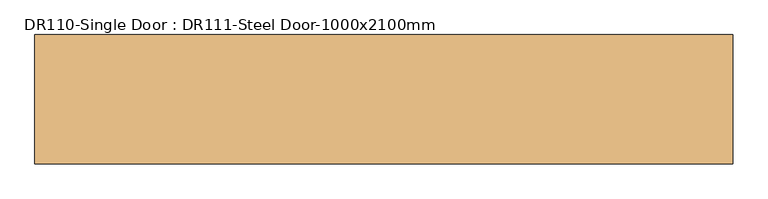
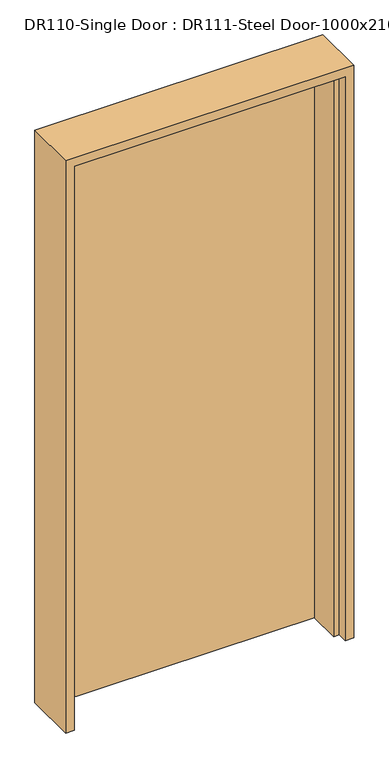
"""IFC4 building model written with IfcOpenShell, lengths in millimetres: door geometry, DR110-Single Door : DR111-Steel Door-1000x2100mm."""

import ifcopenshell
import ifcopenshell.guid

model = None  # the IFC model being written
_history = None  # IfcOwnerHistory: only IFC2X3 demands one
_inside = {}  # id of a spatial element -> (the spatial element, [elements in it])
_under = {}  # id of a project, library or spatial element -> (it, [spatial elements below it])
_declared = {}  # id of a project -> (the project, [libraries it declares])
_typed = {}  # id of a type object -> (the type object, [elements of that type])
_made_of = {}  # id of a material, layer set ... -> (it, [elements and type objects made of it])


def new_model(schema):
    """Start an empty IFC model of exactly this schema.

    Asked for "IFC4X3", IfcOpenShell would pick the latest addendum, in which some entities
    have other attributes; the version numbers below select the first issue.
    IFC2X3 requires an IfcOwnerHistory on every rooted entity: one is made here for all.
    """
    global model, _history
    if schema == "IFC4X3":
        model = ifcopenshell.file(schema_version=(4, 3, 0, 0))
    else:
        model = ifcopenshell.file(schema=schema)
    _inside.clear()
    _under.clear()
    _declared.clear()
    _typed.clear()
    _made_of.clear()
    _history = None
    if model.schema == "IFC2X3":
        org = make("IfcOrganization", Name="unknown")
        user = make(
            "IfcPersonAndOrganization",
            ThePerson=make("IfcPerson", FamilyName="unknown"),
            TheOrganization=org,
        )
        app = make(
            "IfcApplication",
            ApplicationDeveloper=org,
            Version="unknown",
            ApplicationFullName="unknown",
            ApplicationIdentifier="unknown",
        )
        _history = make(
            "IfcOwnerHistory",
            OwningUser=user,
            OwningApplication=app,
            ChangeAction="ADDED",
            CreationDate=0,
        )
    return model


def make(cls, **values):
    """One entity of the class cls with the attributes given. An attribute that is None is left unset."""
    return model.create_entity(
        cls, **{name: value for name, value in values.items() if value is not None}
    )


def rooted(cls, **values):
    """An entity with a GlobalId (a new one), such as an element, a storey or a relation."""
    return make(cls, GlobalId=ifcopenshell.guid.new(), OwnerHistory=_history, **values)


def si_unit(unit_type, name, prefix=None):
    """IfcSIUnit, for example si_unit("LENGTHUNIT", "METRE", prefix="MILLI")."""
    return make("IfcSIUnit", UnitType=unit_type, Prefix=prefix, Name=name)


def assignment(units):
    """IfcUnitAssignment: the units of a project."""
    return None if units is None else make("IfcUnitAssignment", Units=units)


def point(xyz):
    """IfcCartesianPoint."""
    return None if xyz is None else make("IfcCartesianPoint", Coordinates=xyz)


def direction(xyz):
    """IfcDirection."""
    return None if xyz is None else make("IfcDirection", DirectionRatios=xyz)


def frame(location, z_axis=None, x_axis=None):
    """IfcAxis2Placement3D, a coordinate frame: its origin and axes. An axis left out is left unset."""
    return make(
        "IfcAxis2Placement3D",
        Location=point(location),
        Axis=direction(z_axis),
        RefDirection=direction(x_axis),
    )


def origin():
    """The frame at (0, 0, 0) with its axes left unset."""
    return frame((0.0, 0.0, 0.0))


def origin_with_axes():
    """The frame at (0, 0, 0) with the z axis (0, 0, 1) and the x axis (1, 0, 0) written out."""
    return frame((0.0, 0.0, 0.0), z_axis=(0.0, 0.0, 1.0), x_axis=(1.0, 0.0, 0.0))


def place(relative_to, where):
    """IfcLocalPlacement: puts the frame where relative to a parent placement (None: the world)."""
    return make(
        "IfcLocalPlacement", PlacementRelTo=relative_to, RelativePlacement=where
    )


def context(
    kind, dimensions, precision=None, world=None, true_north=None, identifier=None
):
    """IfcGeometricRepresentationContext, for example the 3D "Model" context."""
    return make(
        "IfcGeometricRepresentationContext",
        ContextIdentifier=identifier,
        ContextType=kind,
        CoordinateSpaceDimension=dimensions,
        Precision=precision,
        WorldCoordinateSystem=world,
        TrueNorth=true_north,
    )


def project(units=None, contexts=None):
    """IfcProject with its units and contexts."""
    return rooted(
        "IfcProject",
        Name="project",
        RepresentationContexts=contexts,
        UnitsInContext=assignment(units),
    )


def spatial(cls, under=None, at=None, **own):
    """A site, building, storey or space (cls), placed at a placement, below another one or the project."""
    s = rooted(cls, ObjectPlacement=at, **own)
    if under is not None:
        _under.setdefault(under.id(), (under, []))[1].append(s)
    return s


def polyline(points):
    """IfcPolyline through the points."""
    return make("IfcPolyline", Points=[point(p) for p in points])


def outline(outer, holes=None, kind="AREA"):
    """IfcArbitraryClosedProfileDef: a profile drawn as a closed curve; with holes, ...WithVoids."""
    if holes is None:
        return make("IfcArbitraryClosedProfileDef", ProfileType=kind, OuterCurve=outer)
    return make(
        "IfcArbitraryProfileDefWithVoids",
        ProfileType=kind,
        OuterCurve=outer,
        InnerCurves=holes,
    )


def extrude(swept, where, along, depth):
    """IfcExtrudedAreaSolid: the profile swept, set in the frame where, extruded along a direction by depth."""
    return make(
        "IfcExtrudedAreaSolid",
        SweptArea=swept,
        Position=where,
        ExtrudedDirection=direction(along),
        Depth=depth,
    )


def faces_of(points, faces, orient=None, outer=None):
    """IfcFace entities. A face is a list of loops; a loop is a list of indices into points, from 0.

    orient and outer hold one flag for each loop. By default every Orientation is true, the
    first loop of a face is its IfcFaceOuterBound and the others are IfcFaceBound.
    """
    made = []
    for i, loops in enumerate(faces):
        bounds = []
        for j, loop in enumerate(loops):
            is_outer = j == 0 if outer is None else outer[i][j]
            bounds.append(
                make(
                    "IfcFaceOuterBound" if is_outer else "IfcFaceBound",
                    Bound=make("IfcPolyLoop", Polygon=[points[k] for k in loop]),
                    Orientation=True if orient is None else orient[i][j],
                )
            )
        made.append(make("IfcFace", Bounds=bounds))
    return made


def faceted_brep(points, faces, orient=None, outer=None, voids=None):
    """IfcFacetedBrep: a solid bounded by flat faces; with voids (closed shells), ...WithVoids."""
    shared = [point(p) for p in points]
    hull = make("IfcClosedShell", CfsFaces=faces_of(shared, faces, orient, outer))
    if voids is None:
        return make("IfcFacetedBrep", Outer=hull)
    return make(
        "IfcFacetedBrepWithVoids",
        Outer=hull,
        Voids=[
            make(cls, CfsFaces=faces_of(shared, fs, o, b)) for cls, fs, o, b in voids
        ],
    )


def shape(context_of_items, identifier, shape_type, items):
    """IfcShapeRepresentation: the items that make up one representation, for example the "Body"."""
    return make(
        "IfcShapeRepresentation",
        ContextOfItems=context_of_items,
        RepresentationIdentifier=identifier,
        RepresentationType=shape_type,
        Items=items,
    )


def source(mapping_origin, context_of_items, identifier, shape_type, items):
    """IfcRepresentationMap: a shape defined once, which mapped items show again and again."""
    return make(
        "IfcRepresentationMap",
        MappingOrigin=mapping_origin,
        MappedRepresentation=shape(context_of_items, identifier, shape_type, items),
    )


def transform(
    local_origin,
    x_axis=None,
    y_axis=None,
    z_axis=None,
    scale=None,
    scale2=None,
    scale3=None,
    uniform=True,
):
    """IfcCartesianTransformationOperator3D, or its non-uniform kind. x_axis, y_axis, z_axis: its Axis1, 2, 3."""
    if uniform:
        return make(
            "IfcCartesianTransformationOperator3D",
            Axis1=direction(x_axis),
            Axis2=direction(y_axis),
            LocalOrigin=point(local_origin),
            Scale=scale,
            Axis3=direction(z_axis),
        )
    return make(
        "IfcCartesianTransformationOperator3DnonUniform",
        Axis1=direction(x_axis),
        Axis2=direction(y_axis),
        LocalOrigin=point(local_origin),
        Scale=scale,
        Axis3=direction(z_axis),
        Scale2=scale2,
        Scale3=scale3,
    )


def mapped(mapping_source, mapping_target):
    """IfcMappedItem: shows the shape of a source again, moved by a transform."""
    return make(
        "IfcMappedItem", MappingSource=mapping_source, MappingTarget=mapping_target
    )


def made_of(thing, what):
    """Note that an element or type object is made of a material, layer set ...; save() writes the relation."""
    if what is not None:
        _made_of.setdefault(what.id(), (what, []))[1].append(thing)
    return thing


def element(
    cls,
    number,
    at=None,
    inside=None,
    cuts=None,
    type_object=None,
    material=None,
    context=None,
    identifier="Body",
    shape_type=None,
    held_by="IfcProductDefinitionShape",
    body=None,
    shapes=None,
    **own,
):
    """One element of the class cls, such as IfcWall. Its Tag is "e" and its number.

    at: its placement. inside: the storey or other place that contains it. cuts: it is an
    opening in that element (IfcRelVoidsElement). A single representation is given by context,
    identifier, shape_type and body (its items); several are given by shapes. held_by: the class
    of the entity that holds the representations. save() writes the other relations.
    """
    e = rooted(cls, Tag="e%d" % number, ObjectPlacement=at, **own)
    if body is not None:
        shapes = [shape(context, identifier, shape_type, body)]
    if shapes is not None:
        e.Representation = make(held_by, Representations=shapes)
    if inside is not None:
        _inside.setdefault(inside.id(), (inside, []))[1].append(e)
    if cuts is not None:
        rooted(
            "IfcRelVoidsElement", RelatingBuildingElement=cuts, RelatedOpeningElement=e
        )
    if type_object is not None:
        _typed.setdefault(type_object.id(), (type_object, []))[1].append(e)
    return made_of(e, material)


def aggregate(whole, parts):
    """IfcRelAggregates: a whole, such as a stair, and the parts it consists of."""
    return rooted("IfcRelAggregates", RelatingObject=whole, RelatedObjects=parts)


def save(model, path):
    """Write the relations noted so far, then the file.

    IfcRelAggregates (storeys below a building ...), IfcRelContainedInSpatialStructure (elements
    in a storey), IfcRelDefinesByType, IfcRelAssociatesMaterial and IfcRelDeclares: one each for
    every whole, place, type object, material and project.
    """
    for whole, parts in _under.values():
        aggregate(whole, parts)
    for where, things in _inside.values():
        rooted(
            "IfcRelContainedInSpatialStructure",
            RelatedElements=things,
            RelatingStructure=where,
        )
    for kind, things in _typed.values():
        rooted("IfcRelDefinesByType", RelatedObjects=things, RelatingType=kind)
    for what, things in _made_of.values():
        rooted("IfcRelAssociatesMaterial", RelatedObjects=things, RelatingMaterial=what)
    for by, libraries in _declared.values():
        rooted("IfcRelDeclares", RelatingContext=by, RelatedDefinitions=libraries)
    model.write(path)


def dr110_single_door_dr111_steel_door_1000x2100mm_0699664c(model_context):
    return source(origin(), model_context, "Body", "SolidModel", [
        extrude(outline(polyline([(470.0, 92.5), (470.0, 57.5), (-470.0, 57.5), (-470.0, 92.5), (470.0, 92.5)])), origin_with_axes(), (0.0, 0.0, 1.0), 2070.0),
        faceted_brep([(470.0, 92.5, 0.0), (500.0, 92.5, 0.0), (500.0, -92.5, 0.0), (470.0, -92.5, 0.0), (470.0, -57.5, 0.0), (450.0, -57.5, 0.0), (450.0, 57.5, 0.0), (470.0, 57.5, 0.0), (470.0, 92.5, 2070.0), (-470.0, 92.5, 2070.0), (-470.0, 92.5, 0.0), (-500.0, 92.5, 0.0), (-500.0, 92.5, 2100.0), (500.0, 92.5, 2100.0), (500.0, -92.5, 2100.0), (-500.0, -92.5, 2100.0), (-500.0, -92.5, 0.0), (-470.0, -92.5, 0.0), (-470.0, -92.5, 2070.0), (470.0, -92.5, 2070.0), (470.0, -57.5, 2070.0), (-470.0, -57.5, 2070.0), (-470.0, -57.5, 0.0), (-450.0, -57.5, 0.0), (-450.0, -57.5, 2050.0), (450.0, -57.5, 2050.0), (450.0, 57.5, 2050.0), (-450.0, 57.5, 2050.0), (-450.0, 57.5, 0.0), (-470.0, 57.5, 0.0), (-470.0, 57.5, 2070.0), (470.0, 57.5, 2070.0)], [[[0, 1, 2, 3, 4, 5, 6, 7]], [[1, 0, 8, 9, 10, 11, 12, 13]], [[2, 1, 13, 14]], [[3, 2, 14, 15, 16, 17, 18, 19]], [[4, 3, 19, 20]], [[5, 4, 20, 21, 22, 23, 24, 25]], [[6, 5, 25, 26]], [[7, 6, 26, 27, 28, 29, 30, 31]], [[0, 7, 31, 8]], [[9, 30, 29, 10]], [[10, 29, 28, 23, 22, 17, 16, 11]], [[15, 12, 11, 16]], [[21, 18, 17, 22]], [[27, 24, 23, 28]], [[14, 13, 12, 15]], [[20, 19, 18, 21]], [[26, 25, 24, 27]], [[8, 31, 30, 9]]]),
    ])


if __name__ == "__main__":
    model = new_model("IFC4")
    model_context = context("Model", 3, world=origin())
    ifc_project = project(units=[si_unit("LENGTHUNIT", "METRE", prefix="MILLI")], contexts=[model_context])
    site = spatial("IfcSite", under=ifc_project)
    building = spatial("IfcBuilding", under=site)
    placement = place(None, origin())
    dr110_single_door_dr111_steel_door_1000x2100mm_shape = dr110_single_door_dr111_steel_door_1000x2100mm_0699664c(model_context)
    element("IfcDoor", 1, ObjectType="DR110-Single Door : DR111-Steel Door-1000x2100mm", at=placement, inside=building, context=model_context, shape_type="MappedRepresentation", body=[
        mapped(dr110_single_door_dr111_steel_door_1000x2100mm_shape, transform((0.0, 0.0, 0.0), x_axis=(1.0, 0.0, 0.0), y_axis=(0.0, 1.0, 0.0), z_axis=(0.0, 0.0, 1.0))),
    ])
    save(model, "model.ifc")

# Revit data of these elements
# Type "DR110-Single Door : DR111-Steel Door-1000x2100mm"
#   Description = "DSDSSD"
#   Type Mark = "SD"
#   Analytic Construction = "<None>"
#   프레임 투영 외부. = 25 mm
#   프레임 투영 내부. = 25 mm
#   프레임 폭 = 75 mm
#   Height = 2100 mm
#   Width = 1000 mm
#   Define Thermal Properties by = 1
#   문 패널 = SD1 문 패널
#   문 프레임 = A04AQ098-00002_Steel Door_non FP_single
#   Function = (empty or 0)
#   Wall Closure = (empty or 0)
# Element 1 (IfcDoor, "DR110-Single Door : DR111-Steel Door-1000x2100mm")
#   Materials on its faces: "A04AQ098-00002_Steel Door_non FP_single", "SD1 문 패널"
# Materials
#   "SD1 문 패널": class "금속", colour RGB 247 247 247, transparency 0, Description = "STEEL DOOR (1000Wx2100H)"
#   "A04AQ098-00002_Steel Door_non FP_single": class "금속", colour RGB 247 247 247, transparency 0, Description = "Steel Door", W00) Work Master Code = "A04AQ098-00002", W01) Work Master_Lv1 = "Finishing Work", W02) Work Master_Lv2 = "Door & Window Work", W03) Work Master_Spec.1 = "Steel Door w/ Steel Frame", W04) Work Master_Spec.2 = "Fire Protective Rating: N/A, Single Door", W05) Work Master_Spec.3 = "w/ Hardware & Accessories", Cost = 0
